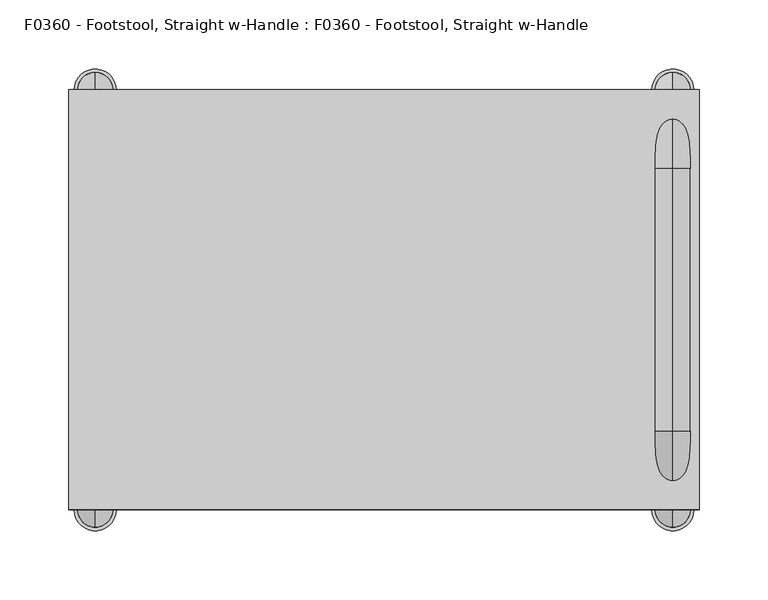
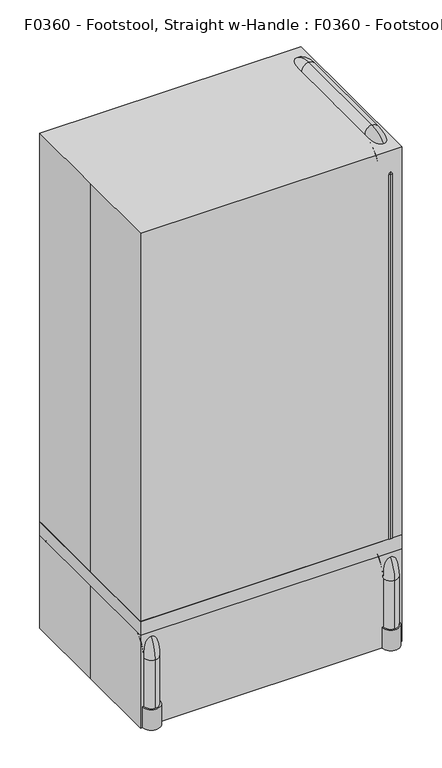
"""IFC4 building model written with IfcOpenShell, lengths in millimetres: proxy geometry, F0360 - Footstool, Straight w-Handle : F0360 - Footstool, Straight w-Handle."""

from ifc_helpers import new_model, si_unit, point, frame, frame_2d, origin, origin_with_axes, place, context, project, spatial, polyline, circle_curve, ellipse_curve, trimmed, segment, composite_curve, outline, extrude, source, transform, mapped, element, save
from ifc_brep_helpers import plane_surface, cylinder_surface, revolved_surface, advanced_brep


def f0360_footstool_straight_w_handle_f0360_footstool_straight_w_84347395(model_context):
    return source(origin(), model_context, "Body", "SolidModel", [
        advanced_brep(
        [(209.4223478, -127.1694395, 196.85), (209.4223478, -152.5694395, 196.85), (209.4223478, -127.1694395, 869.95), (209.4223478, -152.5694395, 869.95), (209.4223478, -95.4194395, 927.1), (209.4223478, -95.4194395, 901.7), (209.4223478, 95.0805605, 901.7), (209.4223478, 95.0805605, 927.1), (209.4223478, 126.8305605, 196.85), (209.4223478, 152.2305605, 196.85), (209.4223478, 152.2305605, 869.95), (209.4223478, 126.8305605, 869.95)],
        [
            (0, 1, circle_curve(frame((209.4223478, -139.8694395, 196.85), z_axis=(0.0, 0.0, -1.0), x_axis=(0.0, -1.0, 0.0)), 12.7)),
            (1, 0, circle_curve(frame((209.4223478, -139.8694395, 196.85), z_axis=(0.0, 0.0, -1.0), x_axis=(0.0, -1.0, 0.0)), 12.7)),
            (0, 2),
            (2, 3, circle_curve(frame((209.4223478, -139.8694395, 869.95), z_axis=(0.0, 0.0, -1.0), x_axis=(0.0, -1.0, 0.0)), 12.7)),
            (3, 1),
            (3, 2, circle_curve(frame((209.4223478, -139.8694395, 869.95), z_axis=(0.0, 0.0, -1.0), x_axis=(0.0, -1.0, 0.0)), 12.7)),
            (4, 5, circle_curve(frame((209.4223478, -95.4194395, 914.4), z_axis=(0.0, 1.0, 0.0), x_axis=(0.0, 0.0, 1.0)), 12.7)),
            (5, 6),
            (6, 7, circle_curve(frame((209.4223478, 95.0805605, 914.4), z_axis=(0.0, -1.0, 0.0), x_axis=(0.0, 0.0, 1.0)), 12.7)),
            (7, 4),
            (5, 4, circle_curve(frame((209.4223478, -95.4194395, 914.4), z_axis=(0.0, 1.0, 0.0), x_axis=(0.0, 0.0, 1.0)), 12.7)),
            (7, 6, circle_curve(frame((209.4223478, 95.0805605, 914.4), z_axis=(0.0, -1.0, 0.0), x_axis=(0.0, 0.0, 1.0)), 12.7)),
            (8, 9, circle_curve(frame((209.4223478, 139.5305605, 196.85), z_axis=(0.0, 0.0, -1.0), x_axis=(0.0, 1.0, 0.0)), 12.7)),
            (9, 8, circle_curve(frame((209.4223478, 139.5305605, 196.85), z_axis=(0.0, 0.0, -1.0), x_axis=(0.0, 1.0, 0.0)), 12.7)),
            (10, 11, circle_curve(frame((209.4223478, 139.5305605, 869.95), z_axis=(0.0, 0.0, -1.0), x_axis=(0.0, 1.0, 0.0)), 12.7)),
            (11, 8),
            (9, 10),
            (11, 10, circle_curve(frame((209.4223478, 139.5305605, 869.95), z_axis=(0.0, 0.0, -1.0), x_axis=(0.0, 1.0, 0.0)), 12.7)),
            (4, 3, circle_curve(frame((209.4223478, -95.4194395, 869.95), z_axis=(1.0, 0.0, 0.0), x_axis=(0.0, -1.0, 0.0)), 57.15)),
            (2, 5, circle_curve(frame((209.4223478, -95.4194395, 869.95), z_axis=(-1.0, 0.0, 0.0), x_axis=(0.0, -1.0, 0.0)), 31.75)),
            (10, 7, circle_curve(frame((209.4223478, 95.0805605, 869.95), z_axis=(1.0, 0.0, 0.0), x_axis=(0.0, 0.0, 1.0)), 57.15)),
            (6, 11, circle_curve(frame((209.4223478, 95.0805605, 869.95), z_axis=(-1.0, 0.0, 0.0), x_axis=(0.0, 0.0, 1.0)), 31.75)),
        ],
        [
            plane_surface(frame((209.4223478, -139.8694395, 196.85), z_axis=(0.0, 0.0, -1.0), x_axis=(1.0, 0.0, 0.0))),
            cylinder_surface(frame((209.4223478, -139.8694395, 196.85), z_axis=(0.0, 0.0, -1.0), x_axis=(0.0, -1.0, 0.0)), 12.7),
            cylinder_surface(frame((209.4223478, -95.4194395, 914.4), z_axis=(0.0, -1.0, 0.0), x_axis=(0.0, 0.0, 1.0)), 12.7),
            plane_surface(frame((209.4223478, 139.5305605, 196.85), z_axis=(0.0, 0.0, -1.0), x_axis=(1.0, 0.0, 0.0))),
            cylinder_surface(frame((209.4223478, 139.5305605, 869.95), z_axis=(0.0, 0.0, 1.0), x_axis=(0.0, 1.0, 0.0)), 12.7),
            revolved_surface(trimmed(ellipse_curve(frame((209.4223478, -139.8694395, 869.95), z_axis=(0.0, 0.0, -1.0), x_axis=(0.0, -1.0, 0.0)), 12.7, 12.7), [point((209.4223478, -127.1694395, 869.95))], [point((209.4223478, -152.5694395, 869.95))], True, "CARTESIAN"), (209.4223478, -95.4194395, 869.95), (-1.0, 0.0, 0.0)),
            revolved_surface(trimmed(ellipse_curve(frame((209.4223478, -139.8694395, 869.95), z_axis=(0.0, 0.0, -1.0), x_axis=(0.0, -1.0, 0.0)), 12.7, 12.7), [point((209.4223478, -152.5694395, 869.95))], [point((209.4223478, -127.1694395, 869.95))], True, "CARTESIAN"), (209.4223478, -95.4194395, 869.95), (-1.0, 0.0, 0.0)),
            revolved_surface(trimmed(ellipse_curve(frame((209.4223478, 95.0805605, 914.4), z_axis=(0.0, -1.0, 0.0), x_axis=(0.0, 0.0, 1.0)), 12.7, 12.7), [point((209.4223478, 95.0805605, 901.7))], [point((209.4223478, 95.0805605, 927.1))], True, "CARTESIAN"), (209.4223478, 95.0805605, 869.95), (-1.0, 0.0, 0.0)),
            revolved_surface(trimmed(ellipse_curve(frame((209.4223478, 95.0805605, 914.4), z_axis=(0.0, -1.0, 0.0), x_axis=(0.0, 0.0, 1.0)), 12.7, 12.7), [point((209.4223478, 95.0805605, 927.1))], [point((209.4223478, 95.0805605, 901.7))], True, "CARTESIAN"), (209.4223478, 95.0805605, 869.95), (-1.0, 0.0, 0.0)),
        ],
        [
            (0, [[1, 2]]),
            (1, [[-1, 3, 4, 5]]),
            (1, [[-2, -5, 6, -3]]),
            (2, [[7, 8, 9, 10]]),
            (2, [[11, -10, 12, -8]]),
            (3, [[13, 14]]),
            (4, [[15, 16, -14, 17]]),
            (4, [[18, -17, -13, -16]]),
            (5, [[19, -4, 20, -7]]),
            (6, [[-20, -6, -19, -11]]),
            (7, [[21, -9, 22, -15]]),
            (8, [[-22, -12, -21, -18]]),
        ],
    ),
        extrude(outline(composite_curve([segment(trimmed(circle_curve(frame_2d((209.55, 152.4)), 15.2941197), [point((224.8441197, 152.4))], [point((194.2558803, 152.4))], False, "CARTESIAN"), True, "CONTINUOUS"), segment(trimmed(circle_curve(frame_2d((209.55, 152.4)), 15.2941197), [point((194.2558803, 152.4))], [point((224.8441197, 152.4))], False, "CARTESIAN"), True, "CONTINUOUS")], self_intersect=False), holes=[composite_curve([segment(trimmed(circle_curve(frame_2d((209.55, 152.4)), 12.7), [point((222.25, 152.4))], [point((196.85, 152.4))], True, "CARTESIAN"), True, "CONTINUOUS"), segment(trimmed(circle_curve(frame_2d((209.55, 152.4)), 12.7), [point((196.85, 152.4))], [point((222.25, 152.4))], True, "CARTESIAN"), True, "CONTINUOUS")], self_intersect=False)]), origin_with_axes(), (0.0, 0.0, 1.0), 38.1),
        extrude(outline(composite_curve([segment(trimmed(circle_curve(frame_2d((-209.55, 152.4)), 15.2941197), [point((-224.8441197, 152.4))], [point((-194.2558803, 152.4))], False, "CARTESIAN"), True, "CONTINUOUS"), segment(trimmed(circle_curve(frame_2d((-209.55, 152.4)), 15.2941197), [point((-194.2558803, 152.4))], [point((-224.8441197, 152.4))], False, "CARTESIAN"), True, "CONTINUOUS")], self_intersect=False), holes=[composite_curve([segment(trimmed(circle_curve(frame_2d((-209.55, 152.4)), 12.7), [point((-222.25, 152.4))], [point((-196.85, 152.4))], True, "CARTESIAN"), True, "CONTINUOUS"), segment(trimmed(circle_curve(frame_2d((-209.55, 152.4)), 12.7), [point((-196.85, 152.4))], [point((-222.25, 152.4))], True, "CARTESIAN"), True, "CONTINUOUS")], self_intersect=False)]), origin_with_axes(), (0.0, 0.0, 1.0), 38.1),
        extrude(outline(composite_curve([segment(trimmed(circle_curve(frame_2d((209.55, -152.4)), 15.2941197), [point((224.8441197, -152.4))], [point((194.2558803, -152.4))], False, "CARTESIAN"), True, "CONTINUOUS"), segment(trimmed(circle_curve(frame_2d((209.55, -152.4)), 15.2941197), [point((194.2558803, -152.4))], [point((224.8441197, -152.4))], False, "CARTESIAN"), True, "CONTINUOUS")], self_intersect=False), holes=[composite_curve([segment(trimmed(circle_curve(frame_2d((209.55, -152.4)), 12.7), [point((222.25, -152.4))], [point((196.85, -152.4))], True, "CARTESIAN"), True, "CONTINUOUS"), segment(trimmed(circle_curve(frame_2d((209.55, -152.4)), 12.7), [point((196.85, -152.4))], [point((222.25, -152.4))], True, "CARTESIAN"), True, "CONTINUOUS")], self_intersect=False)]), origin_with_axes(), (0.0, 0.0, 1.0), 38.1),
        extrude(outline(composite_curve([segment(trimmed(circle_curve(frame_2d((-209.55, -152.4)), 15.2941197), [point((-224.8441197, -152.4))], [point((-194.2558803, -152.4))], False, "CARTESIAN"), True, "CONTINUOUS"), segment(trimmed(circle_curve(frame_2d((-209.55, -152.4)), 15.2941197), [point((-194.2558803, -152.4))], [point((-224.8441197, -152.4))], False, "CARTESIAN"), True, "CONTINUOUS")], self_intersect=False), holes=[composite_curve([segment(trimmed(circle_curve(frame_2d((-209.55, -152.4)), 12.7), [point((-222.25, -152.4))], [point((-196.85, -152.4))], True, "CARTESIAN"), True, "CONTINUOUS"), segment(trimmed(circle_curve(frame_2d((-209.55, -152.4)), 12.7), [point((-196.85, -152.4))], [point((-222.25, -152.4))], True, "CARTESIAN"), True, "CONTINUOUS")], self_intersect=False)]), origin_with_axes(), (0.0, 0.0, 1.0), 38.1),
        advanced_brep(
        [(209.55, -165.1, 0.0), (209.55, -139.7, 0.0), (209.55, -139.7, 127.0), (209.55, -165.1, 127.0), (209.55, -107.95, 184.15), (209.55, -107.95, 158.75), (209.55, 107.95, 158.75), (209.55, 107.95, 184.15), (209.55, 165.1, 127.0), (209.55, 139.7, 127.0), (209.55, 165.1, 0.0), (209.55, 139.7, 0.0)],
        [
            (0, 1, circle_curve(frame((209.55, -152.4, 0.0), z_axis=(0.0, 0.0, -1.0), x_axis=(0.0, 1.0, 0.0)), 12.7)),
            (1, 0, circle_curve(frame((209.55, -152.4, 0.0), z_axis=(0.0, 0.0, -1.0), x_axis=(0.0, 1.0, 0.0)), 12.7)),
            (1, 2),
            (2, 3, circle_curve(frame((209.55, -152.4, 127.0), z_axis=(0.0, 0.0, -1.0), x_axis=(0.0, 1.0, 0.0)), 12.7)),
            (3, 0),
            (3, 2, circle_curve(frame((209.55, -152.4, 127.0), z_axis=(0.0, 0.0, -1.0), x_axis=(0.0, 1.0, 0.0)), 12.7)),
            (4, 3, circle_curve(frame((209.55, -107.95, 127.0), z_axis=(1.0, 0.0, 0.0), x_axis=(0.0, -1.0, 0.0)), 57.15)),
            (2, 5, circle_curve(frame((209.55, -107.95, 127.0), z_axis=(-1.0, 0.0, 0.0), x_axis=(0.0, -1.0, 0.0)), 31.75)),
            (5, 4, circle_curve(frame((209.55, -107.95, 171.45), z_axis=(0.0, -1.0, 0.0), x_axis=(0.0, 0.0, -1.0)), 12.7)),
            (4, 5, circle_curve(frame((209.55, -107.95, 171.45), z_axis=(0.0, -1.0, 0.0), x_axis=(0.0, 0.0, -1.0)), 12.7)),
            (5, 6),
            (6, 7, circle_curve(frame((209.55, 107.95, 171.45), z_axis=(0.0, -1.0, 0.0), x_axis=(0.0, 0.0, -1.0)), 12.7)),
            (7, 4),
            (7, 6, circle_curve(frame((209.55, 107.95, 171.45), z_axis=(0.0, -1.0, 0.0), x_axis=(0.0, 0.0, -1.0)), 12.7)),
            (8, 7, circle_curve(frame((209.55, 107.95, 127.0), z_axis=(1.0, 0.0, 0.0), x_axis=(0.0, 0.0, 1.0)), 57.15)),
            (6, 9, circle_curve(frame((209.55, 107.95, 127.0), z_axis=(-1.0, 0.0, 0.0), x_axis=(0.0, 0.0, 1.0)), 31.75)),
            (9, 8, circle_curve(frame((209.55, 152.4, 127.0), z_axis=(0.0, 0.0, 1.0), x_axis=(0.0, -1.0, 0.0)), 12.7)),
            (8, 9, circle_curve(frame((209.55, 152.4, 127.0), z_axis=(0.0, 0.0, 1.0), x_axis=(0.0, -1.0, 0.0)), 12.7)),
            (10, 11, circle_curve(frame((209.55, 152.4, 0.0), z_axis=(0.0, 0.0, -1.0), x_axis=(0.0, -1.0, 0.0)), 12.7)),
            (11, 10, circle_curve(frame((209.55, 152.4, 0.0), z_axis=(0.0, 0.0, -1.0), x_axis=(0.0, -1.0, 0.0)), 12.7)),
            (9, 11),
            (10, 8),
        ],
        [
            plane_surface(frame((209.55, -152.4, 0.0), z_axis=(0.0, 0.0, -1.0), x_axis=(-1.0, 0.0, 0.0))),
            cylinder_surface(frame((209.55, -152.4, 0.0), z_axis=(0.0, 0.0, -1.0), x_axis=(0.0, 1.0, 0.0)), 12.7),
            revolved_surface(trimmed(ellipse_curve(frame((209.55, -152.4, 127.0), z_axis=(0.0, 0.0, -1.0), x_axis=(0.0, 1.0, 0.0)), 12.7, 12.7), [point((209.55, -139.7, 127.0))], [point((209.55, -165.1, 127.0))], True, "CARTESIAN"), (209.55, -107.95, 127.0), (-1.0, 0.0, 0.0)),
            revolved_surface(trimmed(ellipse_curve(frame((209.55, -152.4, 127.0), z_axis=(0.0, 0.0, -1.0), x_axis=(0.0, 1.0, 0.0)), 12.7, 12.7), [point((209.55, -165.1, 127.0))], [point((209.55, -139.7, 127.0))], True, "CARTESIAN"), (209.55, -107.95, 127.0), (-1.0, 0.0, 0.0)),
            cylinder_surface(frame((209.55, -107.95, 171.45), z_axis=(0.0, -1.0, 0.0), x_axis=(0.0, 0.0, -1.0)), 12.7),
            revolved_surface(trimmed(ellipse_curve(frame((209.55, 107.95, 171.45), z_axis=(0.0, -1.0, 0.0), x_axis=(0.0, 0.0, -1.0)), 12.7, 12.7), [point((209.55, 107.95, 158.75))], [point((209.55, 107.95, 184.15))], True, "CARTESIAN"), (209.55, 107.95, 127.0), (-1.0, 0.0, 0.0)),
            revolved_surface(trimmed(ellipse_curve(frame((209.55, 107.95, 171.45), z_axis=(0.0, -1.0, 0.0), x_axis=(0.0, 0.0, -1.0)), 12.7, 12.7), [point((209.55, 107.95, 184.15))], [point((209.55, 107.95, 158.75))], True, "CARTESIAN"), (209.55, 107.95, 127.0), (-1.0, 0.0, 0.0)),
            plane_surface(frame((209.55, 152.4, 0.0), z_axis=(0.0, 0.0, -1.0), x_axis=(-1.0, 0.0, 0.0))),
            cylinder_surface(frame((209.55, 152.4, 127.0), z_axis=(0.0, 0.0, 1.0), x_axis=(0.0, -1.0, 0.0)), 12.7),
        ],
        [
            (0, [[1, 2]]),
            (1, [[-2, 3, 4, 5]]),
            (1, [[-1, -5, 6, -3]]),
            (2, [[7, -4, 8, 9]]),
            (3, [[-8, -6, -7, 10]]),
            (4, [[-9, 11, 12, 13]]),
            (4, [[-10, -13, 14, -11]]),
            (5, [[15, -12, 16, 17]]),
            (6, [[-16, -14, -15, 18]]),
            (7, [[19, 20]]),
            (8, [[-17, 21, -19, 22]]),
            (8, [[-18, -22, -20, -21]]),
        ],
    ),
        advanced_brep(
        [(-209.55, -139.7, 0.0), (-209.55, -165.1, 0.0), (-209.55, -139.7, 127.0), (-209.55, -165.1, 127.0), (-209.55, -107.95, 184.15), (-209.55, -107.95, 158.75), (-209.55, 107.95, 158.75), (-209.55, 107.95, 184.15), (-209.55, 165.1, 127.0), (-209.55, 139.7, 127.0), (-209.55, 139.7, 0.0), (-209.55, 165.1, 0.0)],
        [
            (0, 1, circle_curve(frame((-209.55, -152.4, 0.0), z_axis=(0.0, 0.0, -1.0), x_axis=(0.0, -1.0, 0.0)), 12.7)),
            (1, 0, circle_curve(frame((-209.55, -152.4, 0.0), z_axis=(0.0, 0.0, -1.0), x_axis=(0.0, -1.0, 0.0)), 12.7)),
            (0, 2),
            (2, 3, circle_curve(frame((-209.55, -152.4, 127.0), z_axis=(0.0, 0.0, -1.0), x_axis=(0.0, -1.0, 0.0)), 12.7)),
            (3, 1),
            (3, 2, circle_curve(frame((-209.55, -152.4, 127.0), z_axis=(0.0, 0.0, -1.0), x_axis=(0.0, -1.0, 0.0)), 12.7)),
            (4, 3, circle_curve(frame((-209.55, -107.95, 127.0), z_axis=(1.0, 0.0, 0.0), x_axis=(0.0, -1.0, 0.0)), 57.15)),
            (2, 5, circle_curve(frame((-209.55, -107.95, 127.0), z_axis=(-1.0, 0.0, 0.0), x_axis=(0.0, -1.0, 0.0)), 31.75)),
            (5, 4, circle_curve(frame((-209.55, -107.95, 171.45), z_axis=(0.0, -1.0, 0.0), x_axis=(0.0, 0.0, 1.0)), 12.7)),
            (4, 5, circle_curve(frame((-209.55, -107.95, 171.45), z_axis=(0.0, -1.0, 0.0), x_axis=(0.0, 0.0, 1.0)), 12.7)),
            (5, 6),
            (6, 7, circle_curve(frame((-209.55, 107.95, 171.45), z_axis=(0.0, -1.0, 0.0), x_axis=(0.0, 0.0, 1.0)), 12.7)),
            (7, 4),
            (7, 6, circle_curve(frame((-209.55, 107.95, 171.45), z_axis=(0.0, -1.0, 0.0), x_axis=(0.0, 0.0, 1.0)), 12.7)),
            (8, 7, circle_curve(frame((-209.55, 107.95, 127.0), z_axis=(1.0, 0.0, 0.0), x_axis=(0.0, 0.0, 1.0)), 57.15)),
            (6, 9, circle_curve(frame((-209.55, 107.95, 127.0), z_axis=(-1.0, 0.0, 0.0), x_axis=(0.0, 0.0, 1.0)), 31.75)),
            (9, 8, circle_curve(frame((-209.55, 152.4, 127.0), z_axis=(0.0, 0.0, 1.0), x_axis=(0.0, 1.0, 0.0)), 12.7)),
            (8, 9, circle_curve(frame((-209.55, 152.4, 127.0), z_axis=(0.0, 0.0, 1.0), x_axis=(0.0, 1.0, 0.0)), 12.7)),
            (10, 11, circle_curve(frame((-209.55, 152.4, 0.0), z_axis=(0.0, 0.0, -1.0), x_axis=(0.0, 1.0, 0.0)), 12.7)),
            (11, 10, circle_curve(frame((-209.55, 152.4, 0.0), z_axis=(0.0, 0.0, -1.0), x_axis=(0.0, 1.0, 0.0)), 12.7)),
            (9, 10),
            (11, 8),
        ],
        [
            plane_surface(frame((-209.55, -152.4, 0.0), z_axis=(0.0, 0.0, -1.0), x_axis=(1.0, 0.0, 0.0))),
            cylinder_surface(frame((-209.55, -152.4, 0.0), z_axis=(0.0, 0.0, -1.0), x_axis=(0.0, -1.0, 0.0)), 12.7),
            revolved_surface(trimmed(ellipse_curve(frame((-209.55, -152.4, 127.0), z_axis=(0.0, 0.0, -1.0), x_axis=(0.0, -1.0, 0.0)), 12.7, 12.7), [point((-209.55, -139.7, 127.0))], [point((-209.55, -165.1, 127.0))], True, "CARTESIAN"), (-209.55, -107.95, 127.0), (-1.0, 0.0, 0.0)),
            revolved_surface(trimmed(ellipse_curve(frame((-209.55, -152.4, 127.0), z_axis=(0.0, 0.0, -1.0), x_axis=(0.0, -1.0, 0.0)), 12.7, 12.7), [point((-209.55, -165.1, 127.0))], [point((-209.55, -139.7, 127.0))], True, "CARTESIAN"), (-209.55, -107.95, 127.0), (-1.0, 0.0, 0.0)),
            cylinder_surface(frame((-209.55, -107.95, 171.45), z_axis=(0.0, -1.0, 0.0), x_axis=(0.0, 0.0, 1.0)), 12.7),
            revolved_surface(trimmed(ellipse_curve(frame((-209.55, 107.95, 171.45), z_axis=(0.0, -1.0, 0.0), x_axis=(0.0, 0.0, 1.0)), 12.7, 12.7), [point((-209.55, 107.95, 158.75))], [point((-209.55, 107.95, 184.15))], True, "CARTESIAN"), (-209.55, 107.95, 127.0), (-1.0, 0.0, 0.0)),
            revolved_surface(trimmed(ellipse_curve(frame((-209.55, 107.95, 171.45), z_axis=(0.0, -1.0, 0.0), x_axis=(0.0, 0.0, 1.0)), 12.7, 12.7), [point((-209.55, 107.95, 184.15))], [point((-209.55, 107.95, 158.75))], True, "CARTESIAN"), (-209.55, 107.95, 127.0), (-1.0, 0.0, 0.0)),
            plane_surface(frame((-209.55, 152.4, 0.0), z_axis=(0.0, 0.0, -1.0), x_axis=(1.0, 0.0, 0.0))),
            cylinder_surface(frame((-209.55, 152.4, 127.0), z_axis=(0.0, 0.0, 1.0), x_axis=(0.0, 1.0, 0.0)), 12.7),
        ],
        [
            (0, [[1, 2]]),
            (1, [[-1, 3, 4, 5]]),
            (1, [[-2, -5, 6, -3]]),
            (2, [[7, -4, 8, 9]]),
            (3, [[-8, -6, -7, 10]]),
            (4, [[-9, 11, 12, 13]]),
            (4, [[-10, -13, 14, -11]]),
            (5, [[15, -12, 16, 17]]),
            (6, [[-16, -14, -15, 18]]),
            (7, [[19, 20]]),
            (8, [[-17, 21, -20, 22]]),
            (8, [[-18, -22, -19, -21]]),
        ],
    ),
        extrude(outline(polyline([(228.6, 152.4), (228.6, -152.4), (-228.6, -152.4), (-228.6, 152.4), (228.6, 152.4)])), frame((0.0, 0.0, 171.45), z_axis=(0.0, 0.0, 1.0), x_axis=(1.0, 0.0, 0.0)), (0.0, 0.0, 1.0), 25.4),
        extrude(outline(polyline([(-228.6, 152.4), (228.6, 152.4), (228.6, -152.4), (-228.6, -152.4), (-228.6, 0.0), (-228.6, 152.4)])), origin_with_axes(), (0.0, 0.0, 1.0), 914.4),
    ])


if __name__ == "__main__":
    model = new_model("IFC4")
    model_context = context("Model", 3, world=origin())
    ifc_project = project(units=[si_unit("LENGTHUNIT", "METRE", prefix="MILLI")], contexts=[model_context])
    site = spatial("IfcSite", under=ifc_project)
    building = spatial("IfcBuilding", under=site)
    placement = place(None, origin())
    f0360_footstool_straight_w_handle_f0360_footstool_straight_w_shape = f0360_footstool_straight_w_handle_f0360_footstool_straight_w_84347395(model_context)
    element("IfcBuildingElementProxy", 1, Name="F0360 - Footstool, Straight w-Handle : F0360 - Footstool, Straight w-Handle", ObjectType="F0360 - Footstool, Straight w-Handle : F0360 - Footstool, Straight w-Handle", at=placement, inside=building, context=model_context, shape_type="MappedRepresentation", body=[
        mapped(f0360_footstool_straight_w_handle_f0360_footstool_straight_w_shape, transform((0.0, 0.0, 0.0), x_axis=(1.0, 0.0, 0.0), y_axis=(0.0, 1.0, 0.0), z_axis=(0.0, 0.0, 1.0))),
    ])
    save(model, "model.ifc")

# Revit data of these elements
# Project information
#   Room Abbreviation = "XMD01"
#   Room Description = "Xray, Mammography (XDM01)"
#   Sheets - Total = "5"
#   Project Issue Date = "Issue Date"
#   Project Status = "Project Status"
#   Client Name = "Owner"
#   Project Address = "Enter address here"
#   Project Name = "Project Name"
#   Project Number = "Project Number"
#   Publication Date = "30-Jan-15"
# Type "F0360 - Footstool, Straight w-Handle : F0360 - Footstool, Straight w-Handle"
#   Watts2 = "0"
#   Watts1 = "0"
#   Unit_Issue = "EA"
#   UTIL_6_Misc = "-"
#   UTIL_5_NonMedGas = "-"
#   UTIL_4_MiscGas = "-"
#   UTIL_3_MedGas = "-"
#   UTIL_2_Elec = "-"
#   UTIL_1_WaterDrain = "-"
#   Nomenclature = "Footstool, Straight w/Handle"
#   NSN = ""
#   Location [instance default] = ""
#   JSN = "F0360"
#   Fund_Source_VA = "-"
#   Fund_Source_Navy = "-"
#   Fund_Source_Army = "-"
#   Fund_Source_AF = "-"
#   ELEC_Volts2 = "0"
#   ELEC_Volts1 = "0"
#   ELEC_Phase2 = "0"
#   ELEC_Phase1 = "0"
#   ELEC_HertzSwitch = "0"
#   ELEC_HertzDependent = "0"
#   ELEC_Hertz = "0"
#   ELEC_Amps2 = "0"
#   ELEC_Amps1 = "0"
#   DetailDescription = ""
#   CAT_VA = "C"
#   CAT_Navy = "C"
#   CAT_IHS = "-"
#   CAT_Army = "C"
#   CAT_AF = "C"
#   BTUperhour = "0"
#   Weight_IP = 0
#   DIM_Width_IP = 1' - 6"
#   DIM_Height_IP = 3' - 0"
#   DIM_Depth_IP = 1' - 0"
# Element 1 (IfcBuildingElementProxy, "F0360 - Footstool, Straight w-Handle : F0360 - Footstool, Straight w-Handle")
#   Materials on its faces: "EquipSpace"
# Materials
#   "EquipSpace": class "Unassigned", colour RGB 221 217 195, transparency 0.5
